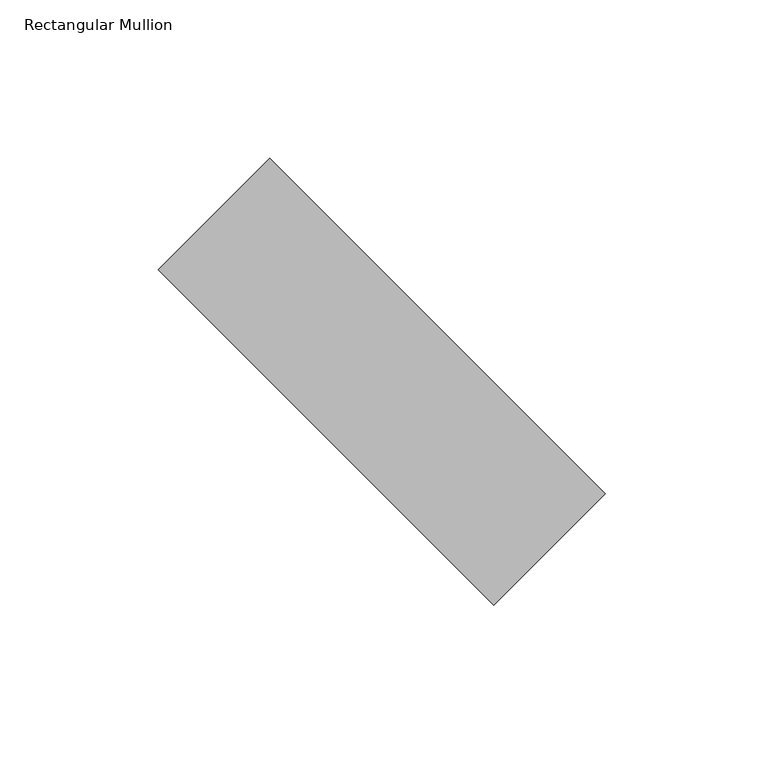
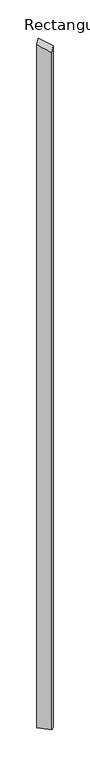
"""IFC4 building model written with IfcOpenShell, lengths in millimetres: member geometry, Rectangular Mullion : tilted mullions."""

from ifc_helpers import new_model, si_unit, origin, place, context, project, spatial, faceted_brep, source, transform, mapped, element, save


def rectangular_mullion_fa86b804(model_context):
    return source(origin(), model_context, "Body", "Brep", [
        faceted_brep([(-35.3553391, 70.7106781, -7999.7416202), (70.7106781, -35.3553391, -7999.7416202), (35.3553391, -70.7106781, -7999.7416202), (-70.7106781, 35.3553391, -7999.7416202), (-70.7106781, 35.3553391, 9.9810707), (-35.3553391, 70.7106781, 55.0394649), (35.3553391, -70.7106781, -55.0394649), (70.7106781, -35.3553391, -9.9810707)], [[[0, 1, 2, 3]], [[4, 5, 0, 3]], [[6, 4, 3, 2]], [[7, 6, 2, 1]], [[5, 7, 1, 0]], [[5, 4, 6, 7]]]),
    ])


if __name__ == "__main__":
    model = new_model("IFC4")
    model_context = context("Model", 3, world=origin())
    ifc_project = project(units=[si_unit("LENGTHUNIT", "METRE", prefix="MILLI")], contexts=[model_context])
    site = spatial("IfcSite", under=ifc_project)
    building = spatial("IfcBuilding", under=site)
    placement = place(None, origin())
    rectangular_mullion_shape = rectangular_mullion_fa86b804(model_context)
    element("IfcMember", 1, ObjectType="Rectangular Mullion : tilted mullions", at=placement, inside=building, context=model_context, shape_type="MappedRepresentation", body=[
        mapped(rectangular_mullion_shape, transform((0.0, 0.0, 0.0), x_axis=(1.0, 0.0, 0.0), y_axis=(0.0, 1.0, 0.0), z_axis=(0.0, 0.0, 1.0))),
    ])
    save(model, "model.ifc")

# Revit data of these elements
# Type "Rectangular Mullion : tilted mullions"
#   built-in parameter 1007304 = 0.492126 (stored number, unit not read)
#   built-in parameter 1007301 = 0.082021 (stored number, unit not read)
#   built-in parameter 1007300 = 0.082021 (stored number, unit not read)
# Element 1 (IfcMember, "Rectangular Mullion : tilted mullions")
#   Materials on its faces: "Aluminum"
# Materials
#   "Aluminum": class "Metal", colour RGB 244 244 244, transparency 0, Description = "Aluminum 6061", Cost = 0
